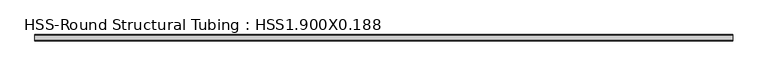
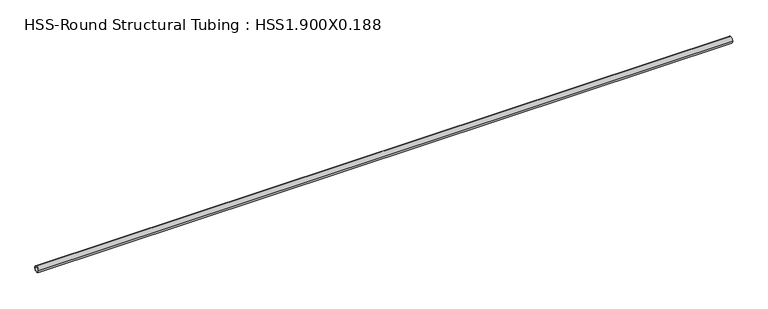
"""IFC4 building model written with IfcOpenShell, lengths in millimetres: member geometry, HSS-Round Structural Tubing : HSS1.900X0.188."""

from ifc_helpers import new_model, si_unit, point, frame, origin, origin_2d, place, context, project, spatial, circle_curve, trimmed, segment, composite_curve, outline, extrude, source, transform, mapped, element, save


def hss_round_structural_tubing_hss1_900x0_188_a00ff317(model_context):
    return source(origin(), model_context, "Body", "SweptSolid", [
        extrude(outline(composite_curve([segment(trimmed(circle_curve(origin_2d(), 24.13), [point((-24.13, 0.0))], [point((24.13, 0.0))], False, "CARTESIAN"), True, "CONTINUOUS"), segment(trimmed(circle_curve(origin_2d(), 24.13), [point((24.13, 0.0))], [point((-24.13, 0.0))], False, "CARTESIAN"), True, "CONTINUOUS")], self_intersect=False), holes=[composite_curve([segment(trimmed(circle_curve(origin_2d(), 19.7104), [point((19.7104, 0.0))], [point((-19.7104, 0.0))], True, "CARTESIAN"), True, "CONTINUOUS"), segment(trimmed(circle_curve(origin_2d(), 19.7104), [point((-19.7104, 0.0))], [point((19.7104, 0.0))], True, "CARTESIAN"), True, "CONTINUOUS")], self_intersect=False)]), frame((-2686.9909588, 0.0, 0.0), z_axis=(1.0, 0.0, 0.0), x_axis=(0.0, 1.0, 0.0)), (0.0, 0.0, 1.0), 5419.7697281),
    ])


if __name__ == "__main__":
    model = new_model("IFC4")
    model_context = context("Model", 3, world=origin())
    ifc_project = project(units=[si_unit("LENGTHUNIT", "METRE", prefix="MILLI")], contexts=[model_context])
    site = spatial("IfcSite", under=ifc_project)
    building = spatial("IfcBuilding", under=site)
    placement = place(None, origin())
    hss_round_structural_tubing_hss1_900x0_188_shape = hss_round_structural_tubing_hss1_900x0_188_a00ff317(model_context)
    element("IfcMember", 1, ObjectType="HSS-Round Structural Tubing : HSS1.900X0.188", at=placement, inside=building, context=model_context, shape_type="MappedRepresentation", body=[
        mapped(hss_round_structural_tubing_hss1_900x0_188_shape, transform((0.0, 0.0, 0.0), x_axis=(1.0, 0.0, 0.0), y_axis=(0.0, 1.0, 0.0), z_axis=(0.0, 0.0, 1.0))),
    ])
    save(model, "model.ifc")

# Revit data of these elements
# Type "HSS-Round Structural Tubing : HSS1.900X0.188"
#   Assembly Code = "B10"
#   t = 4.42 mm
#   W = 3.44
#   Length [instance default] = 1524 mm
#   OD = 48.26 mm
#   A = 0.000608386 m²
#   Structural Material [instance default] = Steel ASTM A500, Grade B, Round
# Element 1 (IfcMember, "HSS-Round Structural Tubing : HSS1.900X0.188")
#   Materials on its faces: "Steel ASTM A500, Grade B, Round"
# Materials
#   "Steel ASTM A500, Grade B, Round": class "Metal", colour RGB 199 199 199, transparency 0, Description = "Carbon steel", Cost = 0
